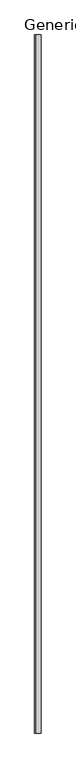
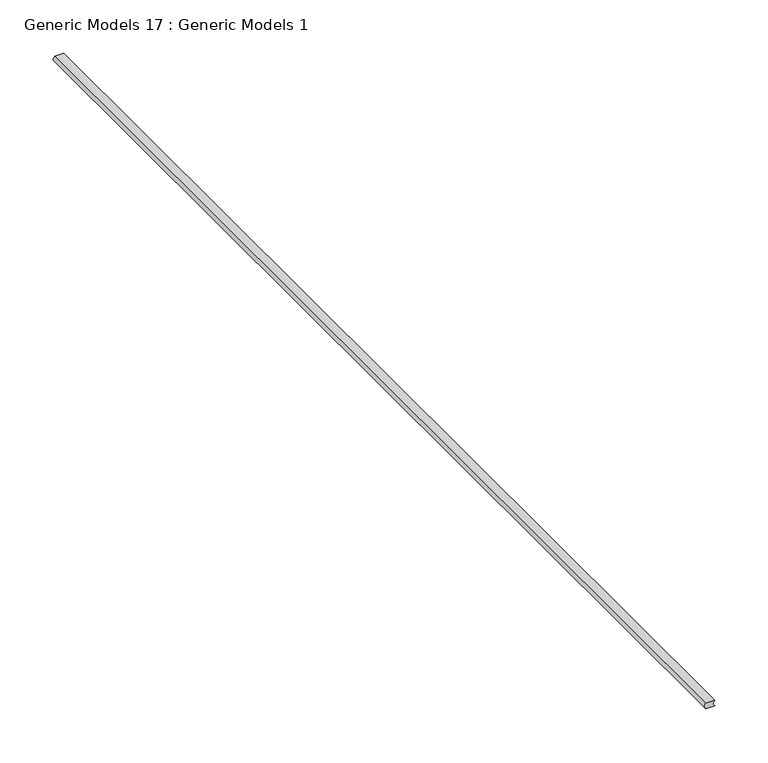
"""IFC4 building model written with IfcOpenShell, lengths in millimetres: proxy geometry, Generic Models 17 : Generic Models 1."""

from ifc_helpers import new_model, si_unit, point, frame, frame_2d, origin, place, context, project, spatial, polyline, circle_curve, trimmed, segment, composite_curve, outline, extrude, source, transform, mapped, element, save


def generic_models_17_generic_models_1_4289aad1(model_context):
    return source(origin(), model_context, "Body", "SweptSolid", [
        extrude(outline(composite_curve([segment(trimmed(circle_curve(frame_2d((3.175, 51021.9897405)), 4.3100275), [point((0.0, 51019.075))], [point((6.35, 51019.075))], True, "CARTESIAN"), True, "CONTINUOUS"), segment(polyline([(6.35, 51019.075), (6.35, 51009.55)]), True, "CONTINUOUS"), segment(trimmed(circle_curve(frame_2d((3.175, 51012.4647405)), 4.3100275), [point((6.35, 51009.55))], [point((0.0, 51009.55))], False, "CARTESIAN"), True, "CONTINUOUS"), segment(polyline([(0.0, 51009.55), (0.0, 51019.075)]), True, "CONTINUOUS")], self_intersect=False)), frame((0.0, 0.0, 0.0), z_axis=(0.0, 1.0, 0.0), x_axis=(0.0, 0.0, 1.0)), (0.0, 0.0, 1.0), 1219.2),
    ])


if __name__ == "__main__":
    model = new_model("IFC4")
    model_context = context("Model", 3, world=origin())
    ifc_project = project(units=[si_unit("LENGTHUNIT", "METRE", prefix="MILLI")], contexts=[model_context])
    site = spatial("IfcSite", under=ifc_project)
    building = spatial("IfcBuilding", under=site)
    placement = place(None, origin())
    generic_models_17_generic_models_1_shape = generic_models_17_generic_models_1_4289aad1(model_context)
    element("IfcBuildingElementProxy", 1, Name="Generic Models 17 : Generic Models 1", ObjectType="Generic Models 17 : Generic Models 1", at=placement, inside=building, context=model_context, shape_type="MappedRepresentation", body=[
        mapped(generic_models_17_generic_models_1_shape, transform((0.0, 0.0, 0.0), x_axis=(1.0, 0.0, 0.0), y_axis=(0.0, 1.0, 0.0), z_axis=(0.0, 0.0, 1.0))),
    ])
    save(model, "model.ifc")

# Revit data of these elements
# Element 1 (IfcBuildingElementProxy, "Generic Models 17 : Generic Models 1")
#   Materials on its faces: "ACOUSTICAL SEALANT"
# Materials
#   "ACOUSTICAL SEALANT": class "Unassigned", colour RGB 120 120 120, transparency 0, Cost = 0
